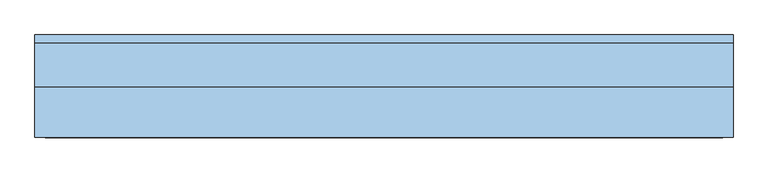
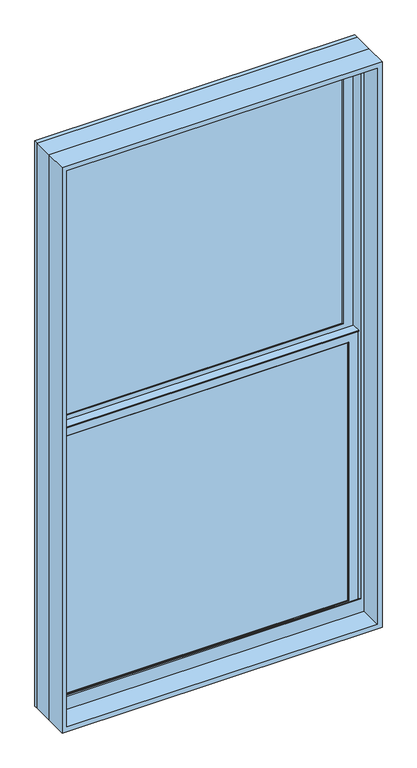
"""IFC4 building model written with IfcOpenShell, lengths in millimetres: window geometry, Window-Double_Hung-Marvin-Essential : ESDH3666."""

from ifc_helpers import new_model, si_unit, frame, origin, place, context, project, spatial, polyline, outline, extrude, faceted_brep, source, transform, mapped, element, save


def window_df7a96b0(model_context):
    return source(origin(), model_context, "Body", "SolidModel", [
        extrude(outline(polyline([(166.1583333, 20.6375), (166.1583333, 15.875), (147.1083333, 15.875), (147.1083333, 20.6375), (166.1583333, 20.6375)])), frame((0.0, 0.0, 527.05), z_axis=(0.0, 0.0, 1.0), x_axis=(1.0, 0.0, 0.0)), (0.0, 0.0, 1.0), 908.05),
        extrude(outline(polyline([(-147.1083333, 20.6375), (-147.1083333, 15.875), (-166.1583333, 15.875), (-166.1583333, 20.6375), (-147.1083333, 20.6375)])), frame((0.0, 0.0, 527.05), z_axis=(0.0, 0.0, 1.0), x_axis=(1.0, 0.0, 0.0)), (0.0, 0.0, 1.0), 908.05),
        extrude(outline(polyline([(469.9, 20.6375), (469.9, 15.875), (-469.9, 15.875), (-469.9, 20.6375), (469.9, 20.6375)])), frame((0.0, 0.0, 971.55), z_axis=(0.0, 0.0, 1.0), x_axis=(1.0, 0.0, 0.0)), (0.0, 0.0, 1.0), 19.05),
        extrude(outline(polyline([(-166.1583333, 46.83125), (-166.1583333, 51.59375), (-147.1083333, 51.59375), (-147.1083333, 46.83125), (-166.1583333, 46.83125)])), frame((0.0, 0.0, 1473.2), z_axis=(0.0, 0.0, 1.0), x_axis=(1.0, 0.0, 0.0)), (0.0, 0.0, 1.0), 908.05),
        extrude(outline(polyline([(147.1083333, 46.83125), (147.1083333, 51.59375), (166.1583333, 51.59375), (166.1583333, 46.83125), (147.1083333, 46.83125)])), frame((0.0, 0.0, 1473.2), z_axis=(0.0, 0.0, 1.0), x_axis=(1.0, 0.0, 0.0)), (0.0, 0.0, 1.0), 908.05),
        extrude(outline(polyline([(-469.9, 46.83125), (-469.9, 51.59375), (469.9, 51.59375), (469.9, 46.83125), (-469.9, 46.83125)])), frame((0.0, 0.0, 1917.7), z_axis=(0.0, 0.0, 1.0), x_axis=(1.0, 0.0, 0.0)), (0.0, 0.0, 1.0), 19.05),
        extrude(outline(polyline([(166.1583333, 20.6375), (147.1083333, 20.6375), (147.1083333, 25.4), (166.1583333, 25.4), (166.1583333, 20.6375)])), frame((0.0, 0.0, 527.05), z_axis=(0.0, 0.0, 1.0), x_axis=(1.0, 0.0, 0.0)), (0.0, 0.0, 1.0), 908.05),
        extrude(outline(polyline([(-147.1083333, 20.6375), (-166.1583333, 20.6375), (-166.1583333, 25.4), (-147.1083333, 25.4), (-147.1083333, 20.6375)])), frame((0.0, 0.0, 527.05), z_axis=(0.0, 0.0, 1.0), x_axis=(1.0, 0.0, 0.0)), (0.0, 0.0, 1.0), 908.05),
        extrude(outline(polyline([(469.9, 20.6375), (-469.9, 20.6375), (-469.9, 25.4), (469.9, 25.4), (469.9, 20.6375)])), frame((0.0, 0.0, 971.55), z_axis=(0.0, 0.0, 1.0), x_axis=(1.0, 0.0, 0.0)), (0.0, 0.0, 1.0), 19.05),
        extrude(outline(polyline([(-166.1583333, 56.35625), (-147.1083333, 56.35625), (-147.1083333, 51.59375), (-166.1583333, 51.59375), (-166.1583333, 56.35625)])), frame((0.0, 0.0, 1473.2), z_axis=(0.0, 0.0, 1.0), x_axis=(1.0, 0.0, 0.0)), (0.0, 0.0, 1.0), 908.05),
        extrude(outline(polyline([(147.1083333, 56.35625), (166.1583333, 56.35625), (166.1583333, 51.59375), (147.1083333, 51.59375), (147.1083333, 56.35625)])), frame((0.0, 0.0, 1473.2), z_axis=(0.0, 0.0, 1.0), x_axis=(1.0, 0.0, 0.0)), (0.0, 0.0, 1.0), 908.05),
        extrude(outline(polyline([(-469.9, 56.35625), (469.9, 56.35625), (469.9, 51.59375), (-469.9, 51.59375), (-469.9, 56.35625)])), frame((0.0, 0.0, 1917.7), z_axis=(0.0, 0.0, 1.0), x_axis=(1.0, 0.0, 0.0)), (0.0, 0.0, 1.0), 19.05),
        faceted_brep([(-496.8875, 5.6780605, 1465.1351748), (-496.8875, 5.6780605, 1460.5), (496.8875, 5.6780605, 1460.5), (496.8875, 5.6780605, 1465.1351748), (-496.8875, 34.8118605, 1465.1351748), (496.8875, 34.8118605, 1465.1351748), (496.8875, 34.8118605, 1460.5), (-496.8875, 34.8118605, 1460.5), (-496.8875, 30.1625, 1460.5), (-496.8875, 30.1625, 500.0625), (-496.8875, 8.9241104, 500.0625), (-496.8875, 8.9241104, 1460.5), (496.8875, 8.9241104, 1460.5), (496.8875, 30.1625, 1460.5), (496.8875, 8.9241104, 500.0625), (496.8875, 30.1625, 500.0625), (-481.0034752, 11.90625, 1446.2034752), (-481.0034752, 30.1625, 1446.2034752), (481.0034752, 30.1625, 1446.2034752), (481.0034752, 11.90625, 1446.2034752), (-464.34375, 10.4662439, 1429.54375), (-464.34375, 11.90625, 1429.54375), (464.34375, 11.90625, 1429.54375), (464.34375, 10.4662439, 1429.54375), (465.8858834, 8.9241104, 1431.0858834), (-465.8858834, 8.9241104, 1431.0858834), (481.0034752, 30.1625, 515.9465248), (481.0034752, 11.90625, 515.9465248), (464.34375, 11.90625, 532.60625), (464.34375, 10.4662439, 532.60625), (465.8858834, 8.9241104, 531.0641166), (-481.0034752, 30.1625, 515.9465248), (-481.0034752, 11.90625, 515.9465248), (-464.34375, 11.90625, 532.60625), (-464.34375, 10.4662439, 532.60625), (-465.8858834, 8.9241104, 531.0641166)], [[[0, 1, 2, 3]], [[4, 5, 6, 7]], [[1, 0, 4, 7, 8, 9, 10, 11]], [[2, 1, 11, 12]], [[7, 6, 13, 8]], [[3, 2, 12, 14, 15, 13, 6, 5]], [[0, 3, 5, 4]], [[16, 17, 18, 19]], [[20, 21, 22, 23]], [[20, 23, 24, 25]], [[19, 18, 26, 27]], [[23, 22, 28, 29]], [[24, 23, 29, 30]], [[27, 26, 31, 32]], [[29, 28, 33, 34]], [[30, 29, 34, 35]], [[15, 14, 10, 9]], [[15, 9, 8, 13], [18, 17, 31, 26]], [[17, 16, 32, 31]], [[16, 19, 27, 32], [22, 21, 33, 28]], [[21, 20, 34, 33]], [[20, 25, 35, 34]], [[10, 14, 12, 11], [25, 24, 30, 35]]]),
        extrude(outline(polyline([(38.5955581, 1446.2125), (33.5778968, 1446.2125), (33.5778968, 1447.8), (39.9405976, 1447.8), (39.9405976, 1446.2125), (61.515625, 1446.2125), (47.6307501, 1442.8975159), (38.5955581, 1442.8975159), (38.5955581, 1446.2125)])), frame((-496.8875, 0.0, 0.0), z_axis=(1.0, 0.0, 0.0), x_axis=(0.0, 1.0, 0.0)), (0.0, 0.0, 1.0), 993.775),
        faceted_brep([(527.05, 0.0, 469.9), (527.05, 0.0, 2438.4), (-527.05, 0.0, 2438.4), (-527.05, 0.0, 469.9), (500.85625, 0.0, 531.01875), (-500.85625, 0.0, 531.01875), (-500.85625, 0.0, 2412.20625), (500.85625, 0.0, 2412.20625), (500.85625, 3.96875, 469.9), (-500.85625, 3.96875, 469.9), (-500.85625, 3.96875, 531.01875), (500.85625, 3.96875, 531.01875), (-527.05, 65.6828125, 469.9), (-500.85625, 65.6828125, 469.9), (500.85625, 65.6828125, 469.9), (527.05, 65.6828125, 469.9), (-527.05, 65.6828125, 2438.4), (527.05, 65.6828125, 2438.4), (500.85625, 65.6828125, 2412.20625), (-500.85625, 65.6828125, 2412.20625)], [[[0, 1, 2, 3], [4, 5, 6, 7]], [[8, 9, 10, 11]], [[5, 4, 11, 10]], [[0, 3, 12, 13, 9, 8, 14, 15]], [[13, 12, 16, 17, 15, 14, 18, 19]], [[13, 19, 6, 5, 10, 9]], [[7, 6, 19, 18]], [[18, 14, 8, 11, 4, 7]], [[1, 0, 15, 17]], [[2, 1, 17, 16]], [[3, 2, 16, 12]]]),
        faceted_brep([(500.85625, 30.1625, 1454.15), (499.26875, 30.1625, 1454.15), (499.26875, 30.1625, 494.2544613), (500.85625, 30.1625, 494.2544613), (-499.26875, 30.1625, 1454.15), (-500.85625, 30.1625, 1454.15), (-500.85625, 30.1625, 494.2544613), (-499.26875, 30.1625, 494.2544613), (499.26875, 63.5, 1454.15), (500.85625, 63.5, 1454.15), (500.85625, 63.5, 487.7743077), (499.26875, 63.5, 487.7743077), (-500.85625, 63.5, 1454.15), (-499.26875, 63.5, 1454.15), (-499.26875, 63.5, 487.7743077), (-500.85625, 63.5, 487.7743077), (512.1108932, 3.96875, 499.3460105), (512.1108932, 3.96875, 469.9), (512.1108932, 65.6828125, 469.9), (512.1108932, 65.6828125, 487.350012), (-512.1108932, 3.96875, 469.9), (-512.1108932, 3.96875, 499.3460105), (-512.1108932, 65.6828125, 487.350012), (-512.1108932, 65.6828125, 469.9), (512.1108932, 78.58125, 484.8428097), (-512.1108932, 78.58125, 484.8428097), (-510.0971252, 68.2348864, 486.8539391), (-492.13135, 68.2348864, 486.8539391), (-492.13135, 65.6828125, 487.350012), (492.13135, 65.6828125, 487.350012), (492.13135, 68.2348864, 486.8539391), (510.0971252, 68.2348864, 486.8539391), (-527.05, 65.6828125, 469.9), (-527.05, 78.5948249, 469.9), (527.05, 78.5948249, 469.9), (527.05, 65.6828125, 469.9), (-527.05, 78.58125, 2438.4), (527.05, 78.58125, 2438.4), (512.1108932, 78.58125, 2423.4608932), (-512.1108932, 78.58125, 2423.4608932), (-527.05, 65.6828125, 2438.4), (-510.0971252, 68.2348864, 2421.4471252), (510.0971252, 68.2348864, 2421.4471252), (492.13135, 68.2348864, 2403.48135), (-492.13135, 68.2348864, 2403.48135), (-492.13135, 65.6828125, 2403.48135), (492.13135, 65.6828125, 2403.48135), (527.05, 65.6828125, 2438.4)], [[[0, 1, 2, 3]], [[4, 5, 6, 7]], [[8, 9, 10, 11]], [[12, 13, 14, 15]], [[1, 8, 11, 2]], [[9, 0, 3, 10]], [[1, 0, 9, 8]], [[5, 4, 13, 12]], [[5, 12, 15, 6]], [[13, 4, 7, 14]], [[16, 17, 18, 19]], [[20, 21, 22, 23]], [[24, 25, 26, 27, 28, 22, 21, 16, 19, 29, 30, 31], [3, 2, 11, 10], [7, 6, 15, 14]], [[17, 16, 21, 20]], [[17, 20, 23, 32, 33, 34, 35, 18]], [[34, 33, 36, 37], [25, 24, 38, 39]], [[33, 32, 40, 36]], [[39, 41, 26, 25]], [[41, 42, 31, 30, 43, 44, 27, 26]], [[44, 45, 28, 27]], [[40, 32, 23, 22, 28, 45, 46, 29, 19, 18, 35, 47]], [[36, 40, 47, 37]], [[39, 38, 42, 41]], [[44, 43, 46, 45]], [[34, 37, 47, 35]], [[42, 38, 24, 31]], [[46, 43, 30, 29]]]),
        extrude(outline(polyline([(477.04375, 11.90625), (-477.04375, 11.90625), (-477.04375, 15.08125), (477.04375, 15.08125), (477.04375, 11.90625)])), frame((0.0, 0.0, 519.90625), z_axis=(0.0, 0.0, 1.0), x_axis=(1.0, 0.0, 0.0)), (0.0, 0.0, 1.0), 922.3375),
        extrude(outline(polyline([(477.04375, 42.8625), (-477.04375, 42.8625), (-477.04375, 46.0375), (477.04375, 46.0375), (477.04375, 42.8625)])), frame((0.0, 0.0, 1466.05625), z_axis=(0.0, 0.0, 1.0), x_axis=(1.0, 0.0, 0.0)), (0.0, 0.0, 1.0), 922.3375),
        faceted_brep([(-464.34375, 31.194477, 1429.54375), (-465.8858834, 32.7366104, 1431.0858834), (465.8858834, 32.7366104, 1431.0858834), (464.34375, 31.194477, 1429.54375), (-464.34375, 30.1625, 1429.54375), (464.34375, 30.1625, 1429.54375), (-496.8875, 32.7366104, 1462.0875), (-496.8875, 30.1625, 1462.0875), (496.8875, 30.1625, 1462.0875), (496.8875, 32.7366104, 1462.0875), (465.8858834, 32.7366104, 531.0641166), (464.34375, 31.194477, 532.60625), (464.34375, 30.1625, 532.60625), (496.8875, 30.1625, 500.0625), (496.8875, 32.7366104, 500.0625), (-465.8858834, 32.7366104, 531.0641166), (-464.34375, 31.194477, 532.60625), (-464.34375, 30.1625, 532.60625), (-496.8875, 30.1625, 500.0625), (-496.8875, 32.7366104, 500.0625)], [[[0, 1, 2, 3]], [[4, 0, 3, 5]], [[6, 7, 8, 9]], [[3, 2, 10, 11]], [[5, 3, 11, 12]], [[9, 8, 13, 14]], [[11, 10, 15, 16]], [[12, 11, 16, 17]], [[14, 13, 18, 19]], [[9, 14, 19, 6], [1, 15, 10, 2]], [[16, 15, 1, 0]], [[17, 16, 0, 4]], [[7, 18, 13, 8], [5, 12, 17, 4]], [[19, 18, 7, 6]]]),
        faceted_brep([(-481.0034752, 42.8625, 2392.3534752), (-481.0034752, 61.11875, 2392.3534752), (481.0034752, 61.11875, 2392.3534752), (481.0034752, 42.8625, 2392.3534752), (-464.34375, 41.4224939, 2375.69375), (-464.34375, 42.8625, 2375.69375), (464.34375, 42.8625, 2375.69375), (464.34375, 41.4224939, 2375.69375), (-465.8858834, 39.8803604, 2377.2358834), (465.8858834, 39.8803604, 2377.2358834), (-496.8875, 61.11875, 2408.2375), (-496.8875, 39.8803604, 2408.2375), (496.8875, 39.8803604, 2408.2375), (496.8875, 61.11875, 2408.2375), (481.0034752, 61.11875, 1462.0965248), (481.0034752, 42.8625, 1462.0965248), (464.34375, 42.8625, 1478.75625), (464.34375, 41.4224939, 1478.75625), (465.8858834, 39.8803604, 1477.2141166), (496.8875, 39.8803604, 1446.2125), (496.8875, 61.11875, 1446.2125), (-481.0034752, 61.11875, 1462.0965248), (-481.0034752, 42.8625, 1462.0965248), (-464.34375, 42.8625, 1478.75625), (-464.34375, 41.4224939, 1478.75625), (-465.8858834, 39.8803604, 1477.2141166), (-496.8875, 39.8803604, 1446.2125), (-496.8875, 61.11875, 1446.2125)], [[[0, 1, 2, 3]], [[4, 5, 6, 7]], [[8, 4, 7, 9]], [[10, 11, 12, 13]], [[3, 2, 14, 15]], [[7, 6, 16, 17]], [[9, 7, 17, 18]], [[13, 12, 19, 20]], [[15, 14, 21, 22]], [[17, 16, 23, 24]], [[18, 17, 24, 25]], [[20, 19, 26, 27]], [[13, 20, 27, 10], [1, 21, 14, 2]], [[22, 21, 1, 0]], [[3, 15, 22, 0], [5, 23, 16, 6]], [[24, 23, 5, 4]], [[25, 24, 4, 8]], [[11, 26, 19, 12], [9, 18, 25, 8]], [[27, 26, 11, 10]]]),
        faceted_brep([(-496.8875, 61.11875, 1446.2125), (-496.8875, 63.6928604, 1446.2125), (496.8875, 63.6928604, 1446.2125), (496.8875, 61.11875, 1446.2125), (-464.34375, 62.150727, 1478.75625), (-464.34375, 61.11875, 1478.75625), (464.34375, 61.11875, 1478.75625), (464.34375, 62.150727, 1478.75625), (-465.8858834, 63.6928604, 1477.2141166), (465.8858834, 63.6928604, 1477.2141166), (496.8875, 63.6928604, 2408.2375), (496.8875, 61.11875, 2408.2375), (464.34375, 61.11875, 2375.69375), (464.34375, 62.150727, 2375.69375), (465.8858834, 63.6928604, 2377.2358834), (-496.8875, 63.6928604, 2408.2375), (-496.8875, 61.11875, 2408.2375), (-464.34375, 61.11875, 2375.69375), (-464.34375, 62.150727, 2375.69375), (-465.8858834, 63.6928604, 2377.2358834)], [[[0, 1, 2, 3]], [[4, 5, 6, 7]], [[8, 4, 7, 9]], [[3, 2, 10, 11]], [[7, 6, 12, 13]], [[9, 7, 13, 14]], [[11, 10, 15, 16]], [[13, 12, 17, 18]], [[14, 13, 18, 19]], [[16, 15, 1, 0]], [[3, 11, 16, 0], [5, 17, 12, 6]], [[18, 17, 5, 4]], [[19, 18, 4, 8]], [[1, 15, 10, 2], [9, 14, 19, 8]]]),
        extrude(outline(polyline([(477.04375, 26.19375), (-477.04375, 26.19375), (-477.04375, 30.1625), (477.04375, 30.1625), (477.04375, 26.19375)])), frame((0.0, 0.0, 519.90625), z_axis=(0.0, 0.0, 1.0), x_axis=(1.0, 0.0, 0.0)), (0.0, 0.0, 1.0), 922.3375),
        extrude(outline(polyline([(477.04375, 57.15), (-477.04375, 57.15), (-477.04375, 61.11875), (477.04375, 61.11875), (477.04375, 57.15)])), frame((0.0, 0.0, 1466.05625), z_axis=(0.0, 0.0, 1.0), x_axis=(1.0, 0.0, 0.0)), (0.0, 0.0, 1.0), 922.3375),
        extrude(outline(polyline([(2438.4, 527.05), (2438.4, -527.05), (469.9, -527.05), (469.9, 527.05), (2438.4, 527.05)]), holes=[polyline([(2422.525, 511.175), (485.775, 511.175), (485.775, -511.175), (2422.525, -511.175), (2422.525, 511.175)])]), frame((0.0, -76.2, 0.0), z_axis=(0.0, 1.0, 0.0), x_axis=(0.0, 0.0, 1.0)), (0.0, 0.0, 1.0), 75.40625),
    ])


if __name__ == "__main__":
    model = new_model("IFC4")
    model_context = context("Model", 3, world=origin())
    ifc_project = project(units=[si_unit("LENGTHUNIT", "METRE", prefix="MILLI")], contexts=[model_context])
    site = spatial("IfcSite", under=ifc_project)
    building = spatial("IfcBuilding", under=site)
    placement = place(None, origin())
    window_shape = window_df7a96b0(model_context)
    element("IfcWindow", 1, ObjectType="Window-Double_Hung-Marvin-Essential : ESDH3666", at=placement, inside=building, context=model_context, shape_type="MappedRepresentation", body=[
        mapped(window_shape, transform((0.0, 0.0, 0.0), x_axis=(1.0, 0.0, 0.0), y_axis=(0.0, 1.0, 0.0), z_axis=(0.0, 0.0, 1.0))),
    ])
    save(model, "model.ifc")

# Revit data of these elements
# Type "Window-Double_Hung-Marvin-Essential : ESDH3666"
#   Type Mark = "87"
#   Window Type = "Essential Double Hung"
#   Product data url = "https://bimobject.com/marvin-windows-and-doors/product/marvin-dhwau"
#   Product Guid = "c4a96547-874c-4385-91dc-a058adc19d98"
#   Frame = "All Ultrex"
#   Egress Window = "Yes"
#   URL = "www.marvin.com"
#   Model = "ESDH3666"
#   Manufacturer = "Marvin Windows and Doors"
#   Label Egress = "EGRESS WDW"
#   Glass Type = "IG Low E II with Argon"
#   Design Pressure = "DP30"
#   Description = "4278 DBHG"
#   Analytic Construction = "<None>"
#   Prairie Corner Width = 0' - 4"
#   Prairie Corner Height = 0' - 4"
#   Egress Width = 3' - 2 9/16"
#   Egress Height = 2' - 10 27/128"
#   Rough Width = 3' - 6"
#   Rough Height = 6' - 6"
#   Nominal Width = 3' - 6"
#   Nominal Height = 6' - 6"
#   Inset to Installation Flange [instance default] = 0' - 1"
#   Height = 6' - 5 1/2"
#   Egress Area = 9.16152 SF
#   Default Head Height = 8' - 0"
#   Width = 3' - 5 1/2"
#   Daylight Area = 17.9321 SF
#   DLO Width = 3' - 0 9/16"
#   DLO Height = 2' - 11 5/16"
#   Muntins Top Sash = yes
#   Lites Wide Top Sash = 3
#   Lites Wide Bottom Sash = 3
#   Lites High Top Sash = 2
#   Lites High Bottom Sash = 2
#   Lite Cut Prairie 9 = no
#   Lite Cut HV Grid = yes
#   Muntins Bottom Sash = yes
#   Label Visibility = no
#   Jamb Extension Visibility = yes
#   Edition number = 1
#   Interior Material = Ultrex-Marvin-Stonewhite
#   Glazing Material = Glass-Marvin-IG Low E II with Argon
#   Cladding Material = Ultrex-Marvin-Pebblegray
#   Wall Closure = (empty or 0)
#   Assembly Code = ""
# Element 1 (IfcWindow, "Window-Double_Hung-Marvin-Essential : ESDH3666")
#   Materials on its faces: "Ultrex-Marvin-Pebblegray", "Ultrex-Marvin-Stonewhite", "Glass-Marvin-IG Low E II with Argon"
# Materials
#   "Ultrex-Marvin-Stonewhite": class "Paint", colour RGB 250 251 245, transparency 0
#   "Glass-Marvin-IG Low E II with Argon": class "Glass", colour RGB 0 128 192, transparency 0.85
#   "Ultrex-Marvin-Pebblegray": class "Paint", colour RGB 189 185 173, transparency 0
